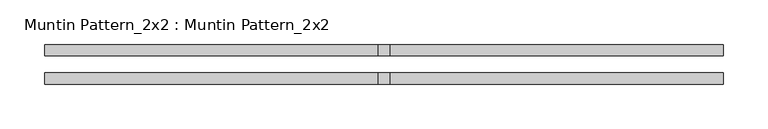
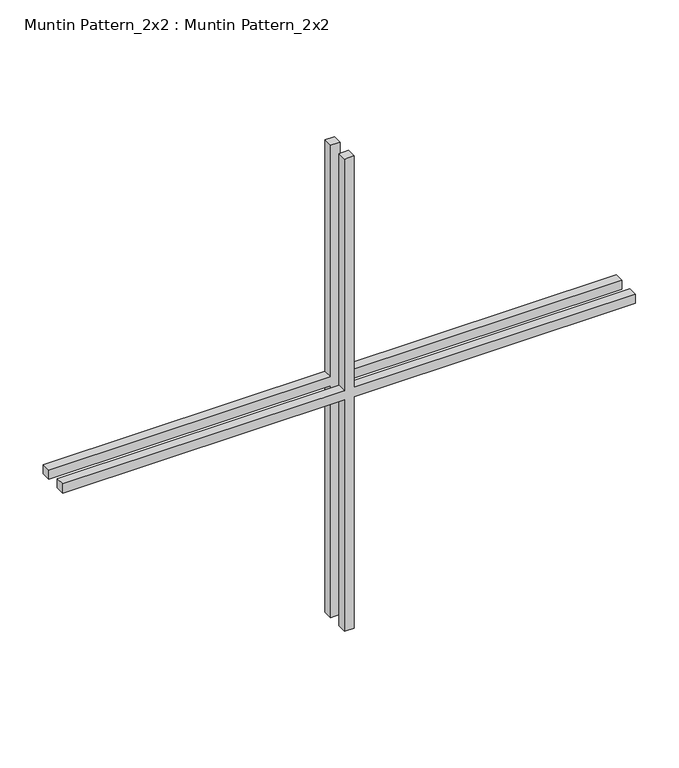
"""IFC4 building model written with IfcOpenShell, lengths in millimetres: proxy geometry, Muntin Pattern_2x2 : Muntin Pattern_2x2."""

from ifc_helpers import new_model, si_unit, frame, origin, place, context, project, spatial, polyline, outline, extrude, source, transform, mapped, element, save


def muntin_pattern_2x2_muntin_pattern_2x2_1ff85060(model_context):
    return source(origin(), model_context, "Body", "SweptSolid", [
        extrude(outline(polyline([(338.1375, -6.35), (338.1375, -381.0), (325.4375, -381.0), (325.4375, -6.35), (0.0, -6.35), (0.0, 6.35), (325.4375, 6.35), (325.4375, 381.0), (338.1375, 381.0), (338.1375, 6.35), (663.575, 6.35), (663.575, -6.35), (338.1375, -6.35)])), frame((0.0, -22.225, 0.0), z_axis=(0.0, 1.0, 0.0), x_axis=(0.0, 0.0, 1.0)), (0.0, 0.0, 1.0), 12.7),
        extrude(outline(polyline([(338.1375, -6.35), (338.1375, -381.0), (325.4375, -381.0), (325.4375, -6.35), (0.0, -6.35), (0.0, 6.35), (325.4375, 6.35), (325.4375, 381.0), (338.1375, 381.0), (338.1375, 6.35), (663.575, 6.35), (663.575, -6.35), (338.1375, -6.35)])), frame((0.0, 9.525, 0.0), z_axis=(0.0, 1.0, 0.0), x_axis=(0.0, 0.0, 1.0)), (0.0, 0.0, 1.0), 12.7),
    ])


if __name__ == "__main__":
    model = new_model("IFC4")
    model_context = context("Model", 3, world=origin())
    ifc_project = project(units=[si_unit("LENGTHUNIT", "METRE", prefix="MILLI")], contexts=[model_context])
    site = spatial("IfcSite", under=ifc_project)
    building = spatial("IfcBuilding", under=site)
    placement = place(None, origin())
    muntin_pattern_2x2_muntin_pattern_2x2_shape = muntin_pattern_2x2_muntin_pattern_2x2_1ff85060(model_context)
    element("IfcBuildingElementProxy", 1, Name="Muntin Pattern_2x2 : Muntin Pattern_2x2", ObjectType="Muntin Pattern_2x2 : Muntin Pattern_2x2", at=placement, inside=building, context=model_context, shape_type="MappedRepresentation", body=[
        mapped(muntin_pattern_2x2_muntin_pattern_2x2_shape, transform((0.0, 0.0, 0.0), x_axis=(1.0, 0.0, 0.0), y_axis=(0.0, 1.0, 0.0), z_axis=(0.0, 0.0, 1.0))),
    ])
    save(model, "model.ifc")

# Revit data of these elements
# Type "Muntin Pattern_2x2 : Muntin Pattern_2x2"
#   Width [instance default] = 4' - 0"
#   Thickness = 0' - 0 1/2"
#   Height [instance default] = 4' - 0"
#   Distance = 0' - 0 3/4"
#   Interior Material [instance default] = none
#   Exterior Material [instance default] = none
#   Default Elevation = 0
# Element 1 (IfcBuildingElementProxy, "Muntin Pattern_2x2 : Muntin Pattern_2x2")
#   Width = 2' - 6"
#   Height = 2' - 2 1/8"
#   Interior Material = Wood - Stained
#   Exterior Material = Clad - White
#   Materials on its faces: "Clad - White", "Wood - Stained"
# Materials
#   "Clad - White": class "Wood", colour RGB 242 242 238, transparency 0, Cost = 0
#   "Wood - Stained": class "Wood", colour RGB 224 178 126, transparency 0, Cost = 0
